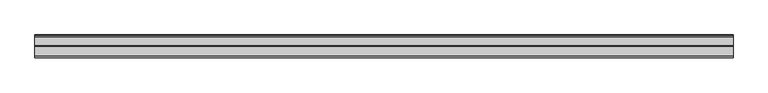
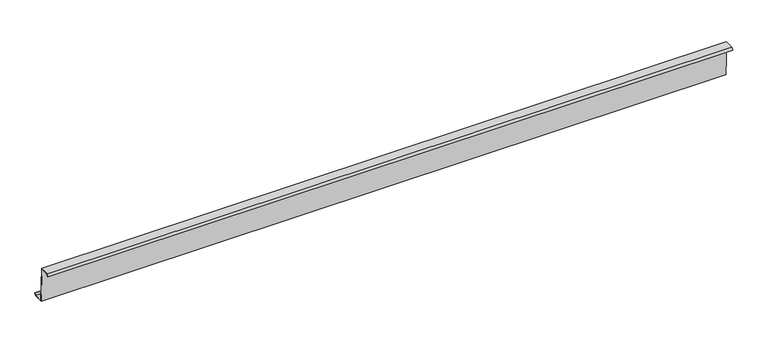
"""IFC4 building model written with IfcOpenShell, lengths in millimetres: proxy geometry, Generic Models 7:Generic Models 1:8:Generic Models 1:8 : Generic Models 7:Generic Models 1:337419:54 : Generic Models 7:Generic Models 1:8:Generic Models 1:8 : Generic Models 7:Generic Models 1:337419:315935."""

from ifc_helpers import new_model, si_unit, frame, origin, place, context, project, spatial, polyline, outline, extrude, source, transform, mapped, element, save


def generic_models_6c65bd77(model_context):
    return source(origin(), model_context, "Body", "SweptSolid", [
        extrude(outline(polyline([(-568396.0172244, 4366.2690904), (-568331.1844159, 4368.9704574), (-568320.7287677, 4118.0348998), (-568259.9660137, 4120.5666812), (-568249.129717, 4134.6307606), (-568246.9290533, 4132.9351612), (-568258.556021, 4117.8448954), (-568323.3888294, 4115.1435284), (-568333.8444776, 4366.079086), (-568394.5769154, 4363.5485678), (-568405.425116, 4349.4690386), (-568407.6441921, 4351.1788246), (-568396.0172244, 4366.2690904)])), frame((591306.0367239, 0.0, 0.0), z_axis=(1.0, 0.0, 0.0), x_axis=(0.0, 1.0, 0.0)), (0.0, 0.0, 1.0), 4876.8),
    ])


if __name__ == "__main__":
    model = new_model("IFC4")
    model_context = context("Model", 3, world=origin())
    ifc_project = project(units=[si_unit("LENGTHUNIT", "METRE", prefix="MILLI")], contexts=[model_context])
    site = spatial("IfcSite", under=ifc_project)
    building = spatial("IfcBuilding", under=site)
    placement = place(None, origin())
    generic_models_shape = generic_models_6c65bd77(model_context)
    element("IfcBuildingElementProxy", 1, Name="Generic Models 7:Generic Models 1:8:Generic Models 1:8 : Generic Models 7:Generic Models 1:337419:54 : Generic Models 7:Generic Models 1:8:Generic Models 1:8 : Generic Models 7:Generic Models 1:337419:315935", ObjectType="Generic Models 7:Generic Models 1:8:Generic Models 1:8 : Generic Models 7:Generic Models 1:337419:54 : Generic Models 7:Generic Models 1:8:Generic Models 1:8 : Generic Models 7:Generic Models 1:337419:315935", at=placement, inside=building, context=model_context, shape_type="MappedRepresentation", body=[
        mapped(generic_models_shape, transform((0.0, 0.0, 0.0), x_axis=(1.0, 0.0, 0.0), y_axis=(0.0, 1.0, 0.0), z_axis=(0.0, 0.0, 1.0))),
    ])
    save(model, "model.ifc")

# Revit data of these elements
# Type "Generic Models 7:Generic Models 1:8:Generic Models 1:8 : Generic Models 7:Generic Models 1:337419:54 : Generic Models 7:Generic Models 1:8:Generic Models 1:8 : Generic Models 7:Generic Models 1:337419:315935"
#   NameOverride = "Generic Models 7:Generic Models 1:8:Generic Models 1:8 : Generic Models 7:Generic Models 1:337419:315935"
#   ObjectTypeOverride = "Generic Models 1:8 : Generic Models 7:Generic Models 1:337419"
#   Reference = "Generic Models 1"
#   Tag = "315935"
# Element 1 (IfcBuildingElementProxy, "Generic Models 7:Generic Models 1:8:Generic Models 1:8 : Generic Models 7:Generic Models 1:337419:54 : Generic Models 7:Generic Models 1:8:Generic Models 1:8 : Generic Models 7:Generic Models 1:337419:315935")
#   Materials on its faces: "ZEE' PURLIN (SEE STRUCT. DWGS)"
# Materials
#   "ZEE' PURLIN (SEE STRUCT. DWGS)": class "Unassigned", colour RGB 210 209 208, transparency 0, Cost = 0
